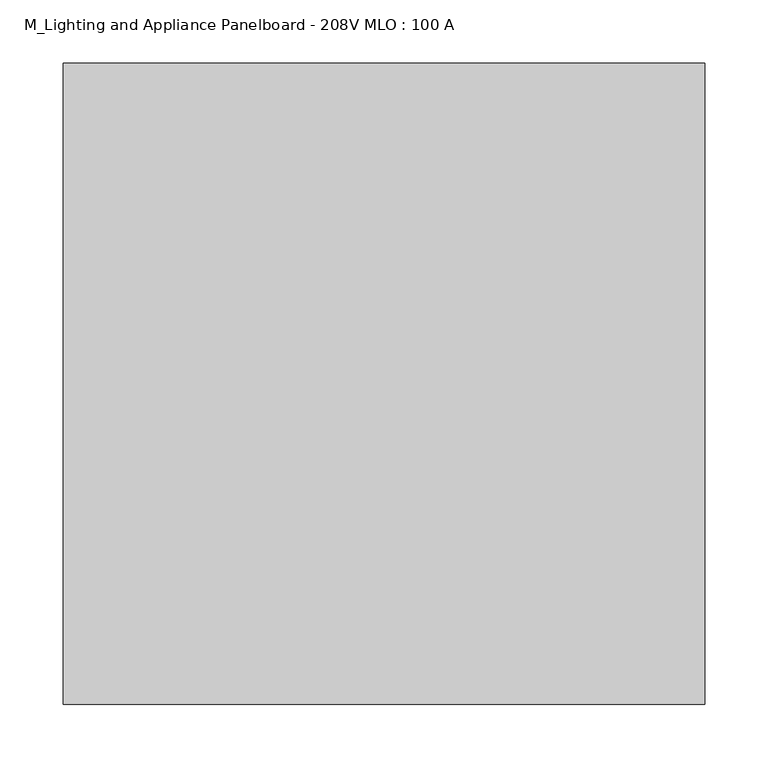
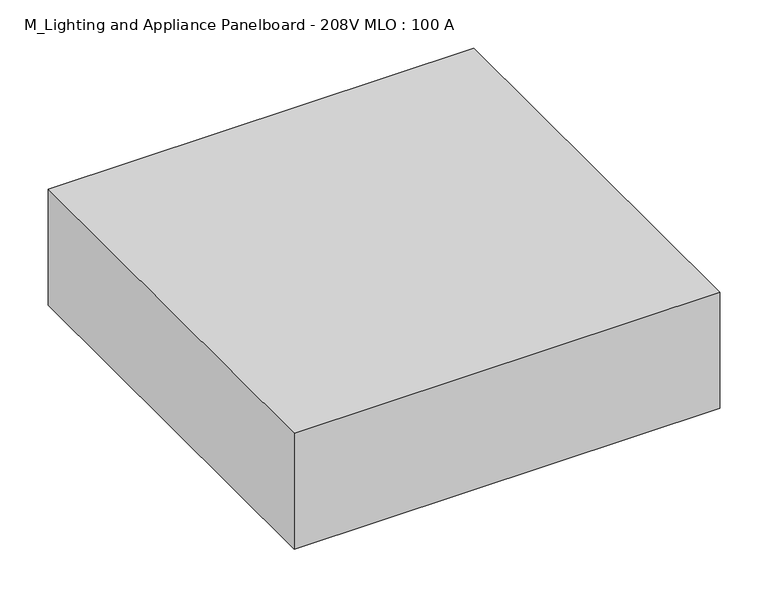
"""IFC4 building model written with IfcOpenShell, lengths in millimetres: proxy geometry, M_Lighting and Appliance Panelboard - 208V MLO : 100 A."""

from ifc_helpers import new_model, si_unit, frame, origin, place, context, project, spatial, polyline, outline, extrude, source, transform, mapped, element, save


def m_lighting_and_appliance_panelboard_208v_mlo_100_a_deb79597(model_context):
    return source(origin(), model_context, "Body", "SweptSolid", [
        extrude(outline(polyline([(254.0, -165.1), (254.0, -673.1), (-254.0, -673.1), (-254.0, -165.1), (254.0, -165.1)])), frame((0.0, 0.0, -146.1), z_axis=(0.0, 0.0, 1.0), x_axis=(1.0, 0.0, 0.0)), (0.0, 0.0, 1.0), 146.1),
    ])


if __name__ == "__main__":
    model = new_model("IFC4")
    model_context = context("Model", 3, world=origin())
    ifc_project = project(units=[si_unit("LENGTHUNIT", "METRE", prefix="MILLI")], contexts=[model_context])
    site = spatial("IfcSite", under=ifc_project)
    building = spatial("IfcBuilding", under=site)
    placement = place(None, origin())
    m_lighting_and_appliance_panelboard_208v_mlo_100_a_shape = m_lighting_and_appliance_panelboard_208v_mlo_100_a_deb79597(model_context)
    element("IfcBuildingElementProxy", 1, Name="M_Lighting and Appliance Panelboard - 208V MLO : 100 A", ObjectType="M_Lighting and Appliance Panelboard - 208V MLO : 100 A", at=placement, inside=building, context=model_context, shape_type="MappedRepresentation", body=[
        mapped(m_lighting_and_appliance_panelboard_208v_mlo_100_a_shape, transform((0.0, 0.0, 0.0), x_axis=(1.0, 0.0, 0.0), y_axis=(0.0, 1.0, 0.0), z_axis=(0.0, 0.0, 1.0))),
    ])
    save(model, "model.ifc")

# Revit data of these elements
# Project information
#   Project Issue Date = "Issue Date"
#   Project Status = "Project Status"
#   Client Name = "Owner"
#   Project Address = "Enter address here"
#   Project Name = "Project Name"
#   Project Number = "Project Number"
# Type "M_Lighting and Appliance Panelboard - 208V MLO : 100 A"
#   built-in parameter 1140081 [instance default] = "Recessed"
#   built-in parameter 1140083 [instance default] = "Type 1"
#   Width = 508 mm
#   built-in parameter 1140082 [instance default] = 100 (stored number, unit not read)
#   Height [instance default] = 508 mm
#   Depth = 146.1 mm
#   Default Elevation = 1200 mm
#   42 Circuit Height = 1041.4 mm
#   30 Circuit Height = 660.4 mm
#   24 Circuit Height = 584.2 mm
#   12 Circuit Height = 508 mm
#   built-in parameter 1140079 [instance default] = 12
#   Load Classification = Other
